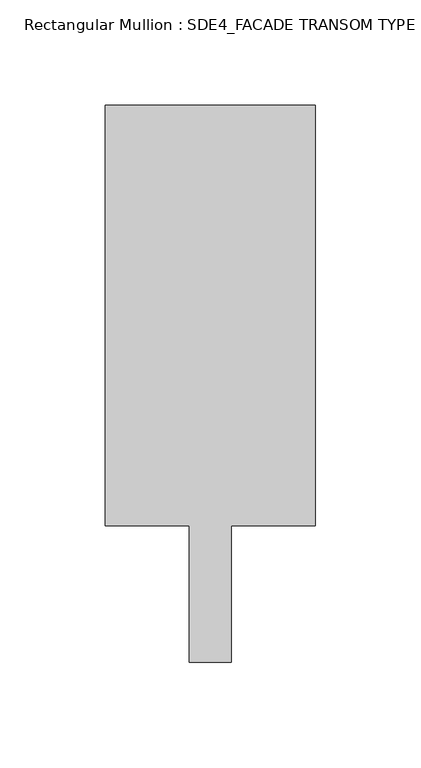
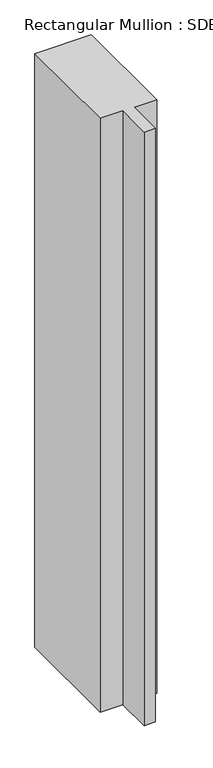
"""IFC4 building model written with IfcOpenShell, lengths in millimetres: member geometry, Rectangular Mullion : SDE4_FACADE TRANSOM TYPE 2."""

from ifc_helpers import new_model, si_unit, frame, origin, place, context, project, spatial, polyline, outline, extrude, source, transform, mapped, element, save


def rectangular_mullion_sde4_facade_transom_type_2_a88ad8f2(model_context):
    return source(origin(), model_context, "Body", "SweptSolid", [
        extrude(outline(polyline([(50.0, 132.5), (50.0, -67.5), (10.0, -67.5), (10.0, -132.5), (-10.0, -132.5), (-10.0, -67.5), (-50.0, -67.5), (-50.0, 132.5), (50.0, 132.5)])), frame((0.0, 0.0, -1110.0), z_axis=(0.0, 0.0, 1.0), x_axis=(1.0, 0.0, 0.0)), (0.0, 0.0, 1.0), 1110.0),
    ])


if __name__ == "__main__":
    model = new_model("IFC4")
    model_context = context("Model", 3, world=origin())
    ifc_project = project(units=[si_unit("LENGTHUNIT", "METRE", prefix="MILLI")], contexts=[model_context])
    site = spatial("IfcSite", under=ifc_project)
    building = spatial("IfcBuilding", under=site)
    placement = place(None, origin())
    rectangular_mullion_sde4_facade_transom_type_2_shape = rectangular_mullion_sde4_facade_transom_type_2_a88ad8f2(model_context)
    element("IfcMember", 1, ObjectType="Rectangular Mullion : SDE4_FACADE TRANSOM TYPE 2", at=placement, inside=building, context=model_context, shape_type="MappedRepresentation", body=[
        mapped(rectangular_mullion_sde4_facade_transom_type_2_shape, transform((0.0, 0.0, 0.0), x_axis=(1.0, 0.0, 0.0), y_axis=(0.0, 1.0, 0.0), z_axis=(0.0, 0.0, 1.0))),
    ])
    save(model, "model.ifc")

# Revit data of these elements
# Type "Rectangular Mullion : SDE4_FACADE TRANSOM TYPE 2"
#   built-in parameter 1007322 = 0.869423 (stored number, unit not read)
#   built-in parameter 1007321 = 0.164042 (stored number, unit not read)
#   built-in parameter 1007320 = 0.164042 (stored number, unit not read)
